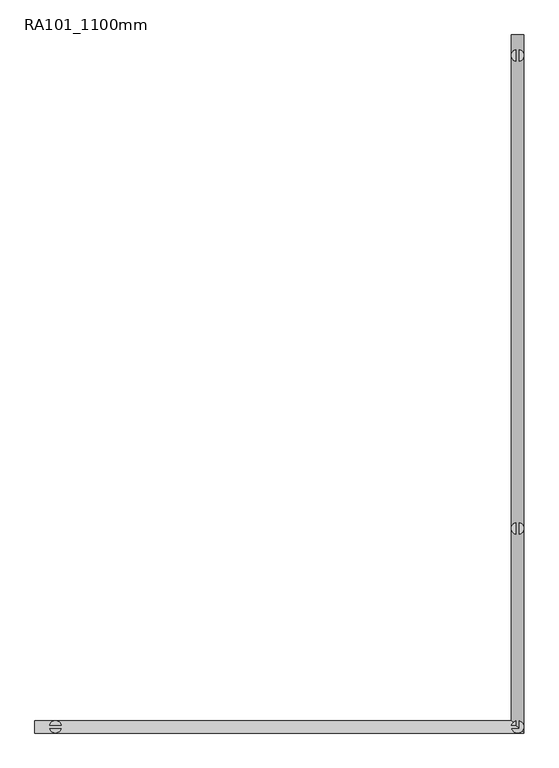
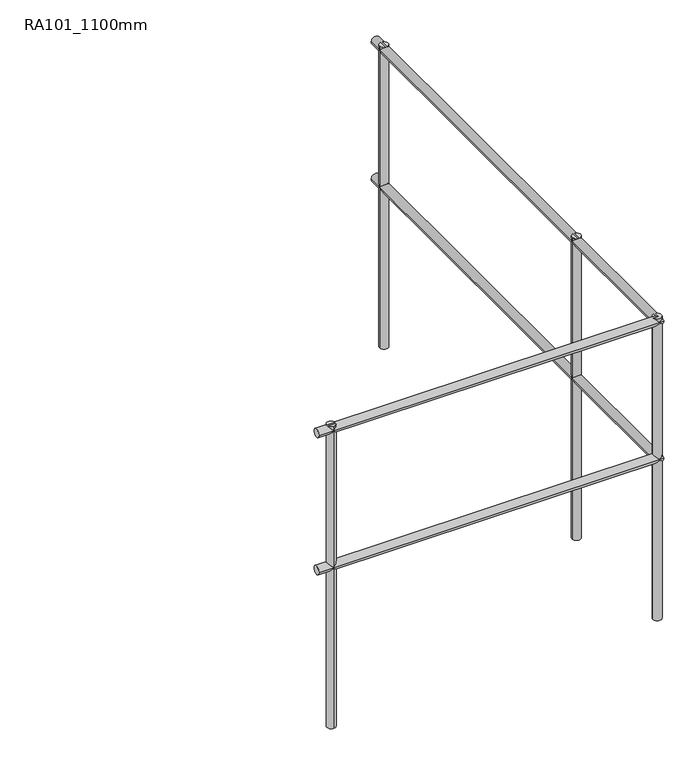
"""IFC4 building model written with IfcOpenShell, lengths in millimetres: railing geometry, RA101_1100mm."""

from ifc_helpers import new_model, si_unit, point, frame, frame_2d, origin, place, context, project, spatial, circle_curve, ellipse_curve, trimmed, segment, composite_curve, outline, extrude, source, transform, mapped, element, save
from ifc_brep_helpers import plane_surface, cylinder_surface, advanced_brep


def ra101_1100mm_da86e9fc(model_context):
    return source(origin(), model_context, "Body", "SolidModel", [
        advanced_brep(
        [(11414.7052251, 14979.5208589, 4745.0), (11384.7052251, 14979.5208589, 4745.0), (10225.0, 13282.0208589, 4745.0), (10225.0, 13312.0208589, 4745.0), (11414.7052251, 13282.0208589, 4745.0), (11384.7052251, 13312.0208589, 4745.0)],
        [
            (0, 1, circle_curve(frame((11399.7052251, 14979.5208589, 4745.0), z_axis=(0.0, 1.0, 0.0), x_axis=(-1.0, 0.0, 0.0)), 15.0)),
            (1, 0, circle_curve(frame((11399.7052251, 14979.5208589, 4745.0), z_axis=(0.0, 1.0, 0.0), x_axis=(-1.0, 0.0, 0.0)), 15.0)),
            (2, 3, circle_curve(frame((10225.0, 13297.0208589, 4745.0), z_axis=(-1.0, 0.0, 0.0), x_axis=(0.0, 1.0, 0.0)), 15.0)),
            (3, 2, circle_curve(frame((10225.0, 13297.0208589, 4745.0), z_axis=(-1.0, 0.0, 0.0), x_axis=(0.0, 1.0, 0.0)), 15.0)),
            (0, 4),
            (4, 5, ellipse_curve(frame((11399.7052251, 13297.0208589, 4745.0), z_axis=(0.7071067811865493, 0.7071067811865457, 0.0), x_axis=(-0.7071067811865457, 0.7071067811865493, 0.0)), 21.2132034, 15.0)),
            (5, 1),
            (5, 4, ellipse_curve(frame((11399.7052251, 13297.0208589, 4745.0), z_axis=(0.7071067811865493, 0.7071067811865457, 0.0), x_axis=(-0.7071067811865457, 0.7071067811865493, 0.0)), 21.2132034, 15.0)),
            (4, 2),
            (3, 5),
        ],
        [
            plane_surface(frame((11399.7052251, 14979.5208589, 4760.0), z_axis=(0.0, 1.0, 0.0), x_axis=(0.0, 0.0, -1.0))),
            plane_surface(frame((10225.0, 13297.0208589, 4760.0), z_axis=(-1.0, 0.0, 0.0), x_axis=(0.0, -1.0, 0.0))),
            cylinder_surface(frame((11399.7052251, 14979.5208589, 4745.0), z_axis=(0.0, 1.0, 0.0), x_axis=(-1.0, 0.0, 0.0)), 15.0),
            cylinder_surface(frame((11399.7052251, 13297.0208589, 4745.0), z_axis=(1.0, 0.0, 0.0), x_axis=(0.0, 1.0, 0.0)), 15.0),
        ],
        [
            (0, [[1, 2]]),
            (1, [[3, 4]]),
            (2, [[-1, 5, 6, 7]]),
            (2, [[-2, -7, 8, -5]]),
            (3, [[-6, 9, -4, 10]]),
            (3, [[-8, -10, -3, -9]]),
        ],
    ),
        advanced_brep(
        [(11414.7052251, 14979.5208589, 5245.0), (11384.7052251, 14979.5208589, 5245.0), (11414.7052251, 13282.0208589, 5245.0), (11384.7052251, 13312.0208589, 5245.0), (10225.0, 13282.0208589, 5245.0), (10225.0, 13312.0208589, 5245.0)],
        [
            (0, 1, circle_curve(frame((11399.7052251, 14979.5208589, 5245.0), z_axis=(0.0, 1.0, 0.0), x_axis=(-1.0, 0.0, 0.0)), 15.0)),
            (1, 0, circle_curve(frame((11399.7052251, 14979.5208589, 5245.0), z_axis=(0.0, 1.0, 0.0), x_axis=(-1.0, 0.0, 0.0)), 15.0)),
            (0, 2),
            (2, 3, ellipse_curve(frame((11399.7052251, 13297.0208589, 5245.0), z_axis=(0.7071067811865493, 0.7071067811865457, 0.0), x_axis=(-0.7071067811865457, 0.7071067811865493, 0.0)), 21.2132034, 15.0)),
            (3, 1),
            (3, 2, ellipse_curve(frame((11399.7052251, 13297.0208589, 5245.0), z_axis=(0.7071067811865493, 0.7071067811865457, 0.0), x_axis=(-0.7071067811865457, 0.7071067811865493, 0.0)), 21.2132034, 15.0)),
            (4, 5, circle_curve(frame((10225.0, 13297.0208589, 5245.0), z_axis=(-1.0, 0.0, 0.0), x_axis=(0.0, 1.0, 0.0)), 15.0)),
            (5, 4, circle_curve(frame((10225.0, 13297.0208589, 5245.0), z_axis=(-1.0, 0.0, 0.0), x_axis=(0.0, 1.0, 0.0)), 15.0)),
            (2, 4),
            (5, 3),
        ],
        [
            plane_surface(frame((11399.7052251, 14979.5208589, 5260.0), z_axis=(0.0, 1.0, 0.0), x_axis=(0.0, 0.0, -1.0))),
            cylinder_surface(frame((11399.7052251, 14979.5208589, 5245.0), z_axis=(0.0, 1.0, 0.0), x_axis=(-1.0, 0.0, 0.0)), 15.0),
            plane_surface(frame((10225.0, 13297.0208589, 5260.0), z_axis=(-1.0, 0.0, 0.0), x_axis=(0.0, -1.0, 0.0))),
            cylinder_surface(frame((11399.7052251, 13297.0208589, 5245.0), z_axis=(1.0, 0.0, 0.0), x_axis=(0.0, 1.0, 0.0)), 15.0),
        ],
        [
            (0, [[1, 2]]),
            (1, [[-1, 3, 4, 5]]),
            (1, [[-2, -5, 6, -3]]),
            (2, [[7, 8]]),
            (3, [[-4, 9, -8, 10]]),
            (3, [[-6, -10, -7, -9]]),
        ],
    ),
        extrude(outline(composite_curve([segment(trimmed(circle_curve(frame_2d((11399.7052251, 13779.5208589)), 15.0), [point((11384.7052251, 13779.5208589))], [point((11414.7052251, 13779.5208589))], False, "CARTESIAN"), True, "CONTINUOUS"), segment(trimmed(circle_curve(frame_2d((11399.7052251, 13779.5208589)), 15.0), [point((11414.7052251, 13779.5208589))], [point((11384.7052251, 13779.5208589))], False, "CARTESIAN"), True, "CONTINUOUS")], self_intersect=False)), frame((0.0, 0.0, 4160.0), z_axis=(0.0, 0.0, 1.0), x_axis=(1.0, 0.0, 0.0)), (0.0, 0.0, 1.0), 1100.0),
        extrude(outline(composite_curve([segment(trimmed(circle_curve(frame_2d((11399.7052251, 13297.0208589)), 15.0), [point((11384.7052251, 13297.0208589))], [point((11414.7052251, 13297.0208589))], False, "CARTESIAN"), True, "CONTINUOUS"), segment(trimmed(circle_curve(frame_2d((11399.7052251, 13297.0208589)), 15.0), [point((11414.7052251, 13297.0208589))], [point((11384.7052251, 13297.0208589))], False, "CARTESIAN"), True, "CONTINUOUS")], self_intersect=False)), frame((0.0, 0.0, 4160.0), z_axis=(0.0, 0.0, 1.0), x_axis=(1.0, 0.0, 0.0)), (0.0, 0.0, 1.0), 1100.0),
        extrude(outline(composite_curve([segment(trimmed(circle_curve(frame_2d((10275.0, 13297.0208589)), 15.0), [point((10275.0, 13312.0208589))], [point((10275.0, 13282.0208589))], False, "CARTESIAN"), True, "CONTINUOUS"), segment(trimmed(circle_curve(frame_2d((10275.0, 13297.0208589)), 15.0), [point((10275.0, 13282.0208589))], [point((10275.0, 13312.0208589))], False, "CARTESIAN"), True, "CONTINUOUS")], self_intersect=False)), frame((0.0, 0.0, 4160.0), z_axis=(0.0, 0.0, 1.0), x_axis=(1.0, 0.0, 0.0)), (0.0, 0.0, 1.0), 1100.0),
        extrude(outline(composite_curve([segment(trimmed(circle_curve(frame_2d((11399.7052251, 14929.5208589)), 15.0), [point((11384.7052251, 14929.5208589))], [point((11414.7052251, 14929.5208589))], False, "CARTESIAN"), True, "CONTINUOUS"), segment(trimmed(circle_curve(frame_2d((11399.7052251, 14929.5208589)), 15.0), [point((11414.7052251, 14929.5208589))], [point((11384.7052251, 14929.5208589))], False, "CARTESIAN"), True, "CONTINUOUS")], self_intersect=False)), frame((0.0, 0.0, 4160.0), z_axis=(0.0, 0.0, 1.0), x_axis=(1.0, 0.0, 0.0)), (0.0, 0.0, 1.0), 1100.0),
    ])


if __name__ == "__main__":
    model = new_model("IFC4")
    model_context = context("Model", 3, world=origin())
    ifc_project = project(units=[si_unit("LENGTHUNIT", "METRE", prefix="MILLI")], contexts=[model_context])
    site = spatial("IfcSite", under=ifc_project)
    building = spatial("IfcBuilding", under=site)
    placement = place(None, origin())
    ra101_1100mm_shape = ra101_1100mm_da86e9fc(model_context)
    element("IfcRailing", 1, ObjectType="RA101_1100mm", at=placement, inside=building, context=model_context, shape_type="MappedRepresentation", body=[
        mapped(ra101_1100mm_shape, transform((0.0, 0.0, 0.0), x_axis=(1.0, 0.0, 0.0), y_axis=(0.0, 1.0, 0.0), z_axis=(0.0, 0.0, 1.0))),
    ])
    save(model, "model.ifc")
